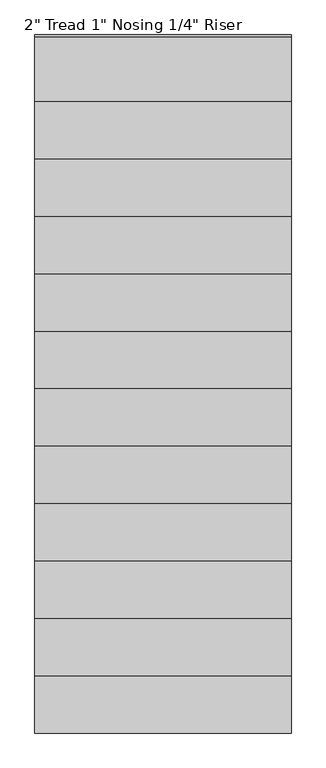
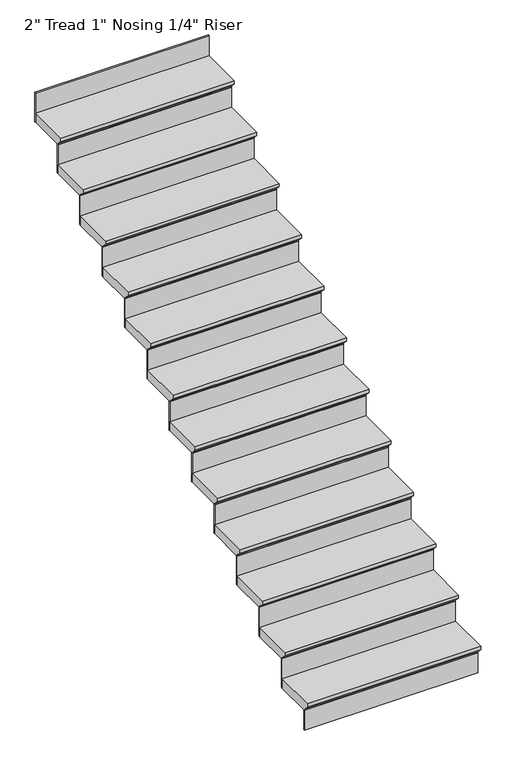
"""IFC4 building model written with IfcOpenShell, lengths in millimetres: stair flight geometry."""

from ifc_helpers import new_model, si_unit, frame, origin, place, context, project, spatial, polyline, outline, extrude, source, transform, mapped, element, save


def stair_flight_42081ac6(model_context):
    return source(origin(), model_context, "Body", "SweptSolid", [
        extrude(outline(polyline([(-12572.2570712, -1934.3076923), (-12343.6570712, -1934.3076923), (-12343.6570712, -1985.1076923), (-12546.8570712, -1985.1076923), (-12546.8570712, -1978.7576923), (-12572.2570712, -1953.3576923), (-12572.2570712, -1934.3076923)])), frame((-25042.4664763, 0.0, 0.0), z_axis=(1.0, 0.0, 0.0), x_axis=(0.0, 1.0, 0.0)), (0.0, 0.0, 1.0), 908.05),
        extrude(outline(polyline([(-24134.4164763, -12540.5070712), (-24134.4164763, -12546.8570712), (-25042.4664763, -12546.8570712), (-25042.4664763, -12540.5070712), (-24134.4164763, -12540.5070712)])), frame((0.0, 0.0, -2095.5), z_axis=(0.0, 0.0, 1.0), x_axis=(1.0, 0.0, 0.0)), (0.0, 0.0, 1.0), 110.3923077),
        extrude(outline(polyline([(-24134.4164763, -12337.3070712), (-24134.4164763, -12343.6570712), (-25042.4664763, -12343.6570712), (-25042.4664763, -12337.3070712), (-24134.4164763, -12337.3070712)])), frame((0.0, 0.0, -1985.1076923), z_axis=(0.0, 0.0, 1.0), x_axis=(1.0, 0.0, 0.0)), (0.0, 0.0, 1.0), 161.1923077),
        extrude(outline(polyline([(-12369.0570712, -1773.1153846), (-12140.4570712, -1773.1153846), (-12140.4570712, -1823.9153846), (-12343.6570712, -1823.9153846), (-12343.6570712, -1817.5653846), (-12369.0570712, -1792.1653846), (-12369.0570712, -1773.1153846)])), frame((-25042.4664763, 0.0, 0.0), z_axis=(1.0, 0.0, 0.0), x_axis=(0.0, 1.0, 0.0)), (0.0, 0.0, 1.0), 908.05),
        extrude(outline(polyline([(-24134.4164763, -12134.1070712), (-24134.4164763, -12140.4570712), (-25042.4664763, -12140.4570712), (-25042.4664763, -12134.1070712), (-24134.4164763, -12134.1070712)])), frame((0.0, 0.0, -1823.9153846), z_axis=(0.0, 0.0, 1.0), x_axis=(1.0, 0.0, 0.0)), (0.0, 0.0, 1.0), 161.1923077),
        extrude(outline(polyline([(-12165.8570712, -1611.9230769), (-11937.2570712, -1611.9230769), (-11937.2570712, -1662.7230769), (-12140.4570712, -1662.7230769), (-12140.4570712, -1656.3730769), (-12165.8570712, -1630.9730769), (-12165.8570712, -1611.9230769)])), frame((-25042.4664763, 0.0, 0.0), z_axis=(1.0, 0.0, 0.0), x_axis=(0.0, 1.0, 0.0)), (0.0, 0.0, 1.0), 908.05),
        extrude(outline(polyline([(-24134.4164763, -11930.9070712), (-24134.4164763, -11937.2570712), (-25042.4664763, -11937.2570712), (-25042.4664763, -11930.9070712), (-24134.4164763, -11930.9070712)])), frame((0.0, 0.0, -1662.7230769), z_axis=(0.0, 0.0, 1.0), x_axis=(1.0, 0.0, 0.0)), (0.0, 0.0, 1.0), 161.1923077),
        extrude(outline(polyline([(-11962.6570712, -1450.7307692), (-11734.0570712, -1450.7307692), (-11734.0570712, -1501.5307692), (-11937.2570712, -1501.5307692), (-11937.2570712, -1495.1807692), (-11962.6570712, -1469.7807692), (-11962.6570712, -1450.7307692)])), frame((-25042.4664763, 0.0, 0.0), z_axis=(1.0, 0.0, 0.0), x_axis=(0.0, 1.0, 0.0)), (0.0, 0.0, 1.0), 908.05),
        extrude(outline(polyline([(-24134.4164763, -11727.7070712), (-24134.4164763, -11734.0570712), (-25042.4664763, -11734.0570712), (-25042.4664763, -11727.7070712), (-24134.4164763, -11727.7070712)])), frame((0.0, 0.0, -1501.5307692), z_axis=(0.0, 0.0, 1.0), x_axis=(1.0, 0.0, 0.0)), (0.0, 0.0, 1.0), 161.1923077),
        extrude(outline(polyline([(-11759.4570712, -1289.5384615), (-11530.8570712, -1289.5384615), (-11530.8570712, -1340.3384615), (-11734.0570712, -1340.3384615), (-11734.0570712, -1333.9884615), (-11759.4570712, -1308.5884615), (-11759.4570712, -1289.5384615)])), frame((-25042.4664763, 0.0, 0.0), z_axis=(1.0, 0.0, 0.0), x_axis=(0.0, 1.0, 0.0)), (0.0, 0.0, 1.0), 908.05),
        extrude(outline(polyline([(-24134.4164763, -11524.5070712), (-24134.4164763, -11530.8570712), (-25042.4664763, -11530.8570712), (-25042.4664763, -11524.5070712), (-24134.4164763, -11524.5070712)])), frame((0.0, 0.0, -1340.3384615), z_axis=(0.0, 0.0, 1.0), x_axis=(1.0, 0.0, 0.0)), (0.0, 0.0, 1.0), 161.1923077),
        extrude(outline(polyline([(-11556.2570712, -1128.3461538), (-11327.6570712, -1128.3461538), (-11327.6570712, -1179.1461538), (-11530.8570712, -1179.1461538), (-11530.8570712, -1172.7961538), (-11556.2570712, -1147.3961538), (-11556.2570712, -1128.3461538)])), frame((-25042.4664763, 0.0, 0.0), z_axis=(1.0, 0.0, 0.0), x_axis=(0.0, 1.0, 0.0)), (0.0, 0.0, 1.0), 908.05),
        extrude(outline(polyline([(-24134.4164763, -11321.3070712), (-24134.4164763, -11327.6570712), (-25042.4664763, -11327.6570712), (-25042.4664763, -11321.3070712), (-24134.4164763, -11321.3070712)])), frame((0.0, 0.0, -1179.1461538), z_axis=(0.0, 0.0, 1.0), x_axis=(1.0, 0.0, 0.0)), (0.0, 0.0, 1.0), 161.1923077),
        extrude(outline(polyline([(-11353.0570712, -967.1538462), (-11124.4570712, -967.1538462), (-11124.4570712, -1017.9538462), (-11327.6570712, -1017.9538462), (-11327.6570712, -1011.6038462), (-11353.0570712, -986.2038462), (-11353.0570712, -967.1538462)])), frame((-25042.4664763, 0.0, 0.0), z_axis=(1.0, 0.0, 0.0), x_axis=(0.0, 1.0, 0.0)), (0.0, 0.0, 1.0), 908.05),
        extrude(outline(polyline([(-24134.4164763, -11118.1070712), (-24134.4164763, -11124.4570712), (-25042.4664763, -11124.4570712), (-25042.4664763, -11118.1070712), (-24134.4164763, -11118.1070712)])), frame((0.0, 0.0, -1017.9538462), z_axis=(0.0, 0.0, 1.0), x_axis=(1.0, 0.0, 0.0)), (0.0, 0.0, 1.0), 161.1923077),
        extrude(outline(polyline([(-11149.8570712, -805.9615385), (-10921.2570712, -805.9615385), (-10921.2570712, -856.7615385), (-11124.4570712, -856.7615385), (-11124.4570712, -850.4115385), (-11149.8570712, -825.0115385), (-11149.8570712, -805.9615385)])), frame((-25042.4664763, 0.0, 0.0), z_axis=(1.0, 0.0, 0.0), x_axis=(0.0, 1.0, 0.0)), (0.0, 0.0, 1.0), 908.05),
        extrude(outline(polyline([(-24134.4164763, -10914.9070712), (-24134.4164763, -10921.2570712), (-25042.4664763, -10921.2570712), (-25042.4664763, -10914.9070712), (-24134.4164763, -10914.9070712)])), frame((0.0, 0.0, -856.7615385), z_axis=(0.0, 0.0, 1.0), x_axis=(1.0, 0.0, 0.0)), (0.0, 0.0, 1.0), 161.1923077),
        extrude(outline(polyline([(-10946.6570712, -644.7692308), (-10718.0570712, -644.7692308), (-10718.0570712, -695.5692308), (-10921.2570712, -695.5692308), (-10921.2570712, -689.2192308), (-10946.6570712, -663.8192308), (-10946.6570712, -644.7692308)])), frame((-25042.4664763, 0.0, 0.0), z_axis=(1.0, 0.0, 0.0), x_axis=(0.0, 1.0, 0.0)), (0.0, 0.0, 1.0), 908.05),
        extrude(outline(polyline([(-24134.4164763, -10711.7070712), (-24134.4164763, -10718.0570712), (-25042.4664763, -10718.0570712), (-25042.4664763, -10711.7070712), (-24134.4164763, -10711.7070712)])), frame((0.0, 0.0, -695.5692308), z_axis=(0.0, 0.0, 1.0), x_axis=(1.0, 0.0, 0.0)), (0.0, 0.0, 1.0), 161.1923077),
        extrude(outline(polyline([(-10743.4570712, -483.5769231), (-10514.8570712, -483.5769231), (-10514.8570712, -534.3769231), (-10718.0570712, -534.3769231), (-10718.0570712, -528.0269231), (-10743.4570712, -502.6269231), (-10743.4570712, -483.5769231)])), frame((-25042.4664763, 0.0, 0.0), z_axis=(1.0, 0.0, 0.0), x_axis=(0.0, 1.0, 0.0)), (0.0, 0.0, 1.0), 908.05),
        extrude(outline(polyline([(-24134.4164763, -10508.5070712), (-24134.4164763, -10514.8570712), (-25042.4664763, -10514.8570712), (-25042.4664763, -10508.5070712), (-24134.4164763, -10508.5070712)])), frame((0.0, 0.0, -534.3769231), z_axis=(0.0, 0.0, 1.0), x_axis=(1.0, 0.0, 0.0)), (0.0, 0.0, 1.0), 161.1923077),
        extrude(outline(polyline([(-10540.2570712, -322.3846154), (-10311.6570712, -322.3846154), (-10311.6570712, -373.1846154), (-10514.8570712, -373.1846154), (-10514.8570712, -366.8346154), (-10540.2570712, -341.4346154), (-10540.2570712, -322.3846154)])), frame((-25042.4664763, 0.0, 0.0), z_axis=(1.0, 0.0, 0.0), x_axis=(0.0, 1.0, 0.0)), (0.0, 0.0, 1.0), 908.05),
        extrude(outline(polyline([(-24134.4164763, -10305.3070712), (-24134.4164763, -10311.6570712), (-25042.4664763, -10311.6570712), (-25042.4664763, -10305.3070712), (-24134.4164763, -10305.3070712)])), frame((0.0, 0.0, -373.1846154), z_axis=(0.0, 0.0, 1.0), x_axis=(1.0, 0.0, 0.0)), (0.0, 0.0, 1.0), 161.1923077),
        extrude(outline(polyline([(-24134.4164763, -10102.1070712), (-24134.4164763, -10108.4570712), (-25042.4664763, -10108.4570712), (-25042.4664763, -10102.1070712), (-24134.4164763, -10102.1070712)])), frame((0.0, 0.0, -211.9923077), z_axis=(0.0, 0.0, 1.0), x_axis=(1.0, 0.0, 0.0)), (0.0, 0.0, 1.0), 161.1923077),
        extrude(outline(polyline([(-10337.0570712, -161.1923077), (-10108.4570712, -161.1923077), (-10108.4570712, -211.9923077), (-10311.6570712, -211.9923077), (-10311.6570712, -205.6423077), (-10337.0570712, -180.2423077), (-10337.0570712, -161.1923077)])), frame((-25042.4664763, 0.0, 0.0), z_axis=(1.0, 0.0, 0.0), x_axis=(0.0, 1.0, 0.0)), (0.0, 0.0, 1.0), 908.05),
    ])


if __name__ == "__main__":
    model = new_model("IFC4")
    model_context = context("Model", 3, world=origin())
    ifc_project = project(units=[si_unit("LENGTHUNIT", "METRE", prefix="MILLI")], contexts=[model_context])
    site = spatial("IfcSite", under=ifc_project)
    building = spatial("IfcBuilding", under=site)
    placement = place(None, origin())
    stair_flight_shape = stair_flight_42081ac6(model_context)
    element("IfcStairFlight", 1, ObjectType="2\" Tread 1\" Nosing 1/4\" Riser", at=placement, inside=building, context=model_context, shape_type="MappedRepresentation", body=[
        mapped(stair_flight_shape, transform((0.0, 0.0, 0.0), x_axis=(1.0, 0.0, 0.0), y_axis=(0.0, 1.0, 0.0), z_axis=(0.0, 0.0, 1.0))),
    ])
    save(model, "model.ifc")
